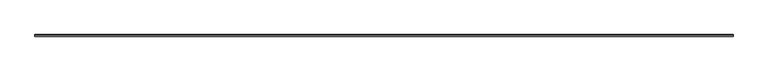
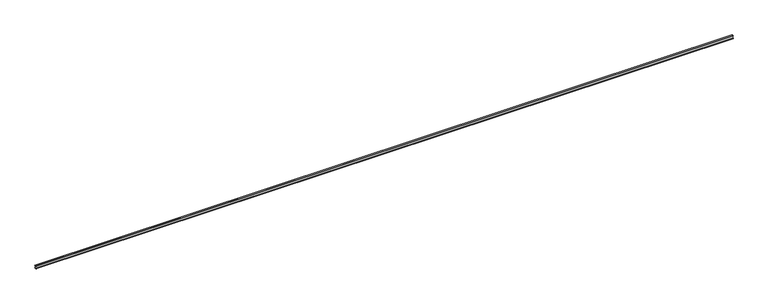
"""IFC4 building model written with IfcOpenShell, lengths in millimetres: proxy geometry, Generic Models 7:Generic Models 1:8:Generic Models 1:8 : Generic Models 7:Generic Models 1:337419:47 : Generic Models 7:Generic Models 1:8:Generic Models 1:8 : Generic Models 7:Generic Models 1:337419:315935."""

from ifc_helpers import new_model, si_unit, frame, origin, place, context, project, spatial, polyline, outline, extrude, source, transform, mapped, element, save


def generic_models_a9e6c8bc(model_context):
    return source(origin(), model_context, "Body", "SweptSolid", [
        extrude(outline(polyline([(-567792.5220098, 8531.5774518), (-567792.8921054, 8540.4597449), (-567628.1928005, 8547.3222159), (-567627.822705, 8538.4399229), (-567707.0635098, 8535.1382227), (-567694.9032277, 8243.291452), (-567615.662423, 8246.5931522), (-567615.2923275, 8237.7108592), (-567779.9916323, 8230.8483882), (-567780.3617279, 8239.7306812), (-567700.867053, 8243.0429593), (-567713.0273351, 8534.88973), (-567792.5220098, 8531.5774518)])), frame((591306.0367239, 0.0, 0.0), z_axis=(1.0, 0.0, 0.0), x_axis=(0.0, 1.0, 0.0)), (0.0, 0.0, 1.0), 75882.0039062),
    ])


if __name__ == "__main__":
    model = new_model("IFC4")
    model_context = context("Model", 3, world=origin())
    ifc_project = project(units=[si_unit("LENGTHUNIT", "METRE", prefix="MILLI")], contexts=[model_context])
    site = spatial("IfcSite", under=ifc_project)
    building = spatial("IfcBuilding", under=site)
    placement = place(None, origin())
    generic_models_shape = generic_models_a9e6c8bc(model_context)
    element("IfcBuildingElementProxy", 1, Name="Generic Models 7:Generic Models 1:8:Generic Models 1:8 : Generic Models 7:Generic Models 1:337419:47 : Generic Models 7:Generic Models 1:8:Generic Models 1:8 : Generic Models 7:Generic Models 1:337419:315935", ObjectType="Generic Models 7:Generic Models 1:8:Generic Models 1:8 : Generic Models 7:Generic Models 1:337419:47 : Generic Models 7:Generic Models 1:8:Generic Models 1:8 : Generic Models 7:Generic Models 1:337419:315935", at=placement, inside=building, context=model_context, shape_type="MappedRepresentation", body=[
        mapped(generic_models_shape, transform((0.0, 0.0, 0.0), x_axis=(1.0, 0.0, 0.0), y_axis=(0.0, 1.0, 0.0), z_axis=(0.0, 0.0, 1.0))),
    ])
    save(model, "model.ifc")

# Revit data of these elements
# Type "Generic Models 7:Generic Models 1:8:Generic Models 1:8 : Generic Models 7:Generic Models 1:337419:47 : Generic Models 7:Generic Models 1:8:Generic Models 1:8 : Generic Models 7:Generic Models 1:337419:315935"
#   NameOverride = "Generic Models 7:Generic Models 1:8:Generic Models 1:8 : Generic Models 7:Generic Models 1:337419:315935"
#   ObjectTypeOverride = "Generic Models 1:8 : Generic Models 7:Generic Models 1:337419"
#   Reference = "Generic Models 1"
#   Tag = "315935"
# Element 1 (IfcBuildingElementProxy, "Generic Models 7:Generic Models 1:8:Generic Models 1:8 : Generic Models 7:Generic Models 1:337419:47 : Generic Models 7:Generic Models 1:8:Generic Models 1:8 : Generic Models 7:Generic Models 1:337419:315935")
#   Materials on its faces: "STRUCTURAL STEEL - SEE STRUCT. DWGS"
# Materials
#   "STRUCTURAL STEEL - SEE STRUCT. DWGS": class "Metal", colour RGB 189 187 185, transparency 0, Description = "Structural steel 50ksi", Cost = 0
